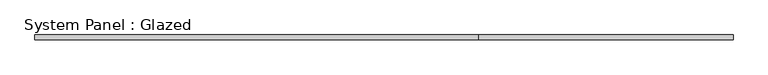
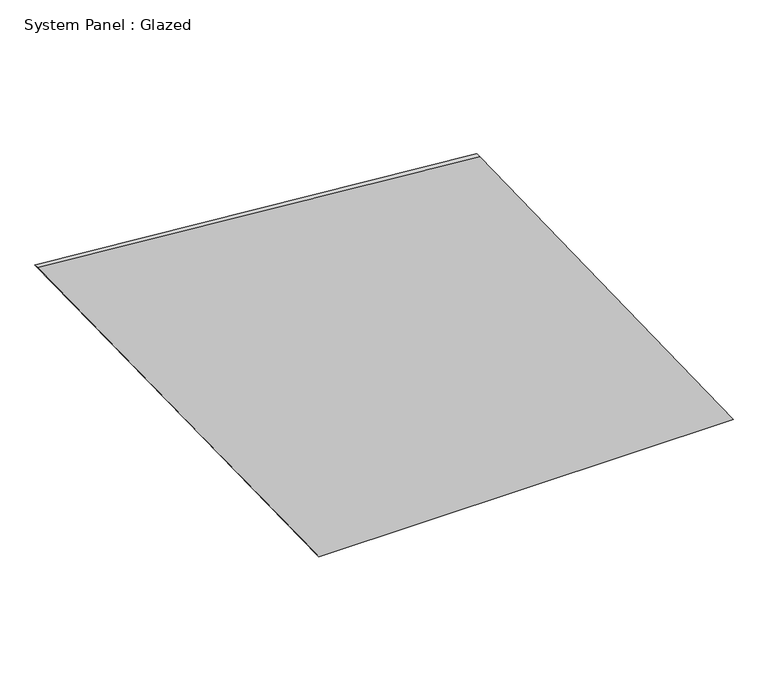
"""IFC4 building model written with IfcOpenShell, lengths in millimetres: plate geometry, System Panel : Glazed."""

from ifc_helpers import new_model, si_unit, frame, origin, place, context, project, spatial, polyline, outline, extrude, source, transform, mapped, element, save


def system_panel_glazed_2e6e4282(model_context):
    return source(origin(), model_context, "Body", "SweptSolid", [
        extrude(outline(polyline([(0.0, -338.8991765), (0.0, 1769.8447666), (1869.0084775, 480.5231567), (2057.2903553, -1769.8447666), (0.0, -338.8991765)])), frame((0.0, -49.5, 0.0), z_axis=(0.0, 1.0, 0.0), x_axis=(0.0, 0.0, 1.0)), (0.0, 0.0, 1.0), 25.0),
    ])


if __name__ == "__main__":
    model = new_model("IFC4")
    model_context = context("Model", 3, world=origin())
    ifc_project = project(units=[si_unit("LENGTHUNIT", "METRE", prefix="MILLI")], contexts=[model_context])
    site = spatial("IfcSite", under=ifc_project)
    building = spatial("IfcBuilding", under=site)
    placement = place(None, origin())
    system_panel_glazed_shape = system_panel_glazed_2e6e4282(model_context)
    element("IfcPlate", 1, ObjectType="System Panel : Glazed", at=placement, inside=building, context=model_context, shape_type="MappedRepresentation", body=[
        mapped(system_panel_glazed_shape, transform((0.0, 0.0, 0.0), x_axis=(1.0, 0.0, 0.0), y_axis=(0.0, 1.0, 0.0), z_axis=(0.0, 0.0, 1.0))),
    ])
    save(model, "model.ifc")

# Revit data of these elements
# Element 1 (IfcPlate, "System Panel : Glazed")
#   Materials on its faces: "Glass, Clear Glazing"
# Materials
#   "Glass, Clear Glazing": class "Glass", colour RGB 247 249 248, transparency 0.85, Description = "Clear glazing", Cost = 0
